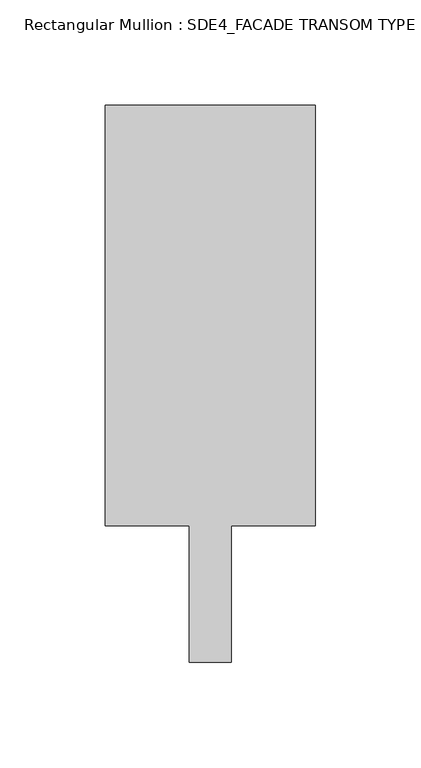
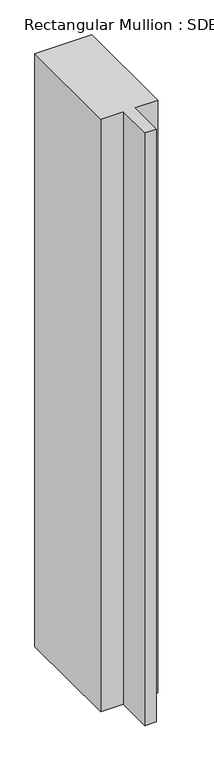
"""IFC4 building model written with IfcOpenShell, lengths in millimetres: member geometry, Rectangular Mullion : SDE4_FACADE TRANSOM TYPE 2."""

from ifc_helpers import new_model, si_unit, frame, origin, place, context, project, spatial, polyline, outline, extrude, source, transform, mapped, element, save


def rectangular_mullion_sde4_facade_transom_type_2_d9762d9f(model_context):
    return source(origin(), model_context, "Body", "SweptSolid", [
        extrude(outline(polyline([(50.0, 132.5), (50.0, -67.5), (10.0, -67.5), (10.0, -132.5), (-10.0, -132.5), (-10.0, -67.5), (-50.0, -67.5), (-50.0, 132.5), (50.0, 132.5)])), frame((0.0, 0.0, -1100.0), z_axis=(0.0, 0.0, 1.0), x_axis=(1.0, 0.0, 0.0)), (0.0, 0.0, 1.0), 1100.0),
    ])


if __name__ == "__main__":
    model = new_model("IFC4")
    model_context = context("Model", 3, world=origin())
    ifc_project = project(units=[si_unit("LENGTHUNIT", "METRE", prefix="MILLI")], contexts=[model_context])
    site = spatial("IfcSite", under=ifc_project)
    building = spatial("IfcBuilding", under=site)
    placement = place(None, origin())
    rectangular_mullion_sde4_facade_transom_type_2_shape = rectangular_mullion_sde4_facade_transom_type_2_d9762d9f(model_context)
    element("IfcMember", 1, ObjectType="Rectangular Mullion : SDE4_FACADE TRANSOM TYPE 2", at=placement, inside=building, context=model_context, shape_type="MappedRepresentation", body=[
        mapped(rectangular_mullion_sde4_facade_transom_type_2_shape, transform((0.0, 0.0, 0.0), x_axis=(1.0, 0.0, 0.0), y_axis=(0.0, 1.0, 0.0), z_axis=(0.0, 0.0, 1.0))),
    ])
    save(model, "model.ifc")

# Revit data of these elements
# Type "Rectangular Mullion : SDE4_FACADE TRANSOM TYPE 2"
#   built-in parameter 1007322 = 0.869423 (stored number, unit not read)
#   built-in parameter 1007321 = 0.164042 (stored number, unit not read)
#   built-in parameter 1007320 = 0.164042 (stored number, unit not read)
